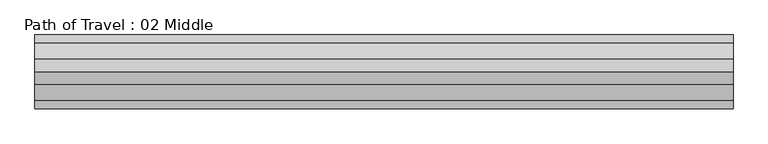
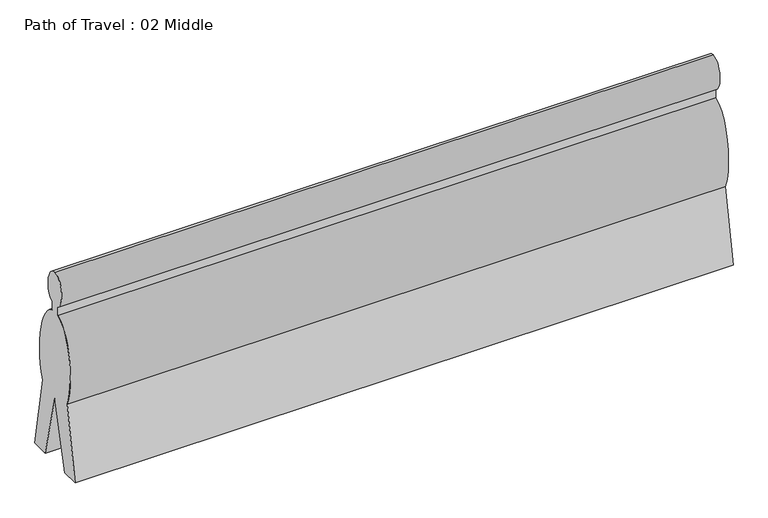
"""IFC4 building model written with IfcOpenShell, lengths in millimetres: proxy geometry, Path of Travel : 02 Middle."""

from ifc_helpers import new_model, si_unit, point, frame, origin, place, context, project, spatial, ellipse_curve, trimmed, source, transform, mapped, element, save
from ifc_brep_helpers import plane_surface, extruded_surface, advanced_brep


def path_of_travel_02_middle_da6d7806(model_context):
    return source(origin(), model_context, "Body", "AdvancedBrep", [
        advanced_brep(
        [(227.5554837, 0.0, 1727.2), (227.5554837, 42.9018657, 1436.6534209), (227.5554837, 42.9018657, 1363.4763406), (227.5554837, 184.1186263, 643.4144547), (227.5554837, 297.5699544, 0.0), (227.5554837, 145.6574193, 0.0), (227.5554837, 0.0, 584.2), (227.5554837, -145.6574193, 0.0), (227.5554837, -297.5699544, 0.0), (227.5554837, -184.1186263, 643.4144547), (227.5554837, -42.9018657, 1363.4763406), (227.5554837, -42.9018657, 1436.6534209), (5866.3554837, 0.0, 1727.2), (5866.3554837, -42.9018657, 1436.6534209), (5866.3554837, -42.9018657, 1363.4763406), (5866.3554837, -184.1186263, 643.4144547), (5866.3554837, -297.5699544, 0.0), (5866.3554837, -145.6574193, 0.0), (5866.3554837, 0.0, 584.2), (5866.3554837, 145.6574193, 0.0), (5866.3554837, 297.5699544, 0.0), (5866.3554837, 184.1186263, 643.4144547), (5866.3554837, 42.9018657, 1363.4763406), (5866.3554837, 42.9018657, 1436.6534209)],
        [
            (0, 1, ellipse_curve(frame((227.5554837, 0.0, 1574.8), z_axis=(-1.0, 0.0, 0.0), x_axis=(0.0, 0.0, 1.0)), 152.4, 101.6)),
            (1, 2),
            (2, 3, ellipse_curve(frame((227.5554837, 0.0, 914.4), z_axis=(-1.0, 0.0, 0.0), x_axis=(0.0, 0.0, -1.0)), 457.2, 228.6)),
            (3, 4),
            (4, 5),
            (5, 6),
            (6, 7),
            (7, 8),
            (8, 9),
            (9, 10, ellipse_curve(frame((227.5554837, 0.0, 914.4), z_axis=(-1.0, 0.0, 0.0), x_axis=(0.0, 0.0, -1.0)), 457.2, 228.6)),
            (10, 11),
            (11, 0, ellipse_curve(frame((227.5554837, 0.0, 1574.8), z_axis=(-1.0, 0.0, 0.0), x_axis=(0.0, 0.0, 1.0)), 152.4, 101.6)),
            (12, 13, ellipse_curve(frame((5866.3554837, 0.0, 1574.8), z_axis=(1.0, 0.0, 0.0), x_axis=(0.0, 0.0, 1.0)), 152.4, 101.6)),
            (13, 14),
            (14, 15, ellipse_curve(frame((5866.3554837, 0.0, 914.4), z_axis=(1.0, 0.0, 0.0), x_axis=(0.0, 0.0, -1.0)), 457.2, 228.6)),
            (15, 16),
            (16, 17),
            (17, 18),
            (18, 19),
            (19, 20),
            (20, 21),
            (21, 22, ellipse_curve(frame((5866.3554837, 0.0, 914.4), z_axis=(1.0, 0.0, 0.0), x_axis=(0.0, 0.0, -1.0)), 457.2, 228.6)),
            (22, 23),
            (23, 12, ellipse_curve(frame((5866.3554837, 0.0, 1574.8), z_axis=(1.0, 0.0, 0.0), x_axis=(0.0, 0.0, 1.0)), 152.4, 101.6)),
            (0, 12),
            (23, 1),
            (22, 2),
            (21, 3),
            (20, 4),
            (19, 5),
            (18, 6),
            (17, 7),
            (16, 8),
            (15, 9),
            (14, 10),
            (13, 11),
        ],
        [
            plane_surface(frame((227.5554837, 0.0, 0.0), z_axis=(-1.0, 0.0, 0.0), x_axis=(0.0, 0.0, 1.0))),
            plane_surface(frame((5866.3554837, 0.0, 0.0), z_axis=(1.0, 0.0, 0.0), x_axis=(0.0, 0.0, 1.0))),
            extruded_surface(trimmed(ellipse_curve(frame((5866.3554837, 0.0, 1574.8), z_axis=(-1.0, 0.0, 0.0), x_axis=(0.0, 0.0, 1.0)), 152.4, 101.6), [point((5866.3554837, 0.0, 1727.2))], [point((5866.3554837, 42.9018657, 1436.6534209))], True, "CARTESIAN"), (-5638.8, 0.0, 0.0), 5638.8),
            plane_surface(frame((227.5554837, 42.9018657, 1436.6534209), z_axis=(0.0, 1.0, 0.0), x_axis=(1.0, 0.0, 0.0))),
            extruded_surface(trimmed(ellipse_curve(frame((5866.3554837, 0.0, 914.4), z_axis=(-1.0, 0.0, 0.0), x_axis=(0.0, 0.0, -1.0)), 457.2, 228.6), [point((5866.3554837, 42.9018657, 1363.4763406))], [point((5866.3554837, 184.1186263, 643.4144547))], True, "CARTESIAN"), (-5638.8, 0.0, 0.0), 5638.8),
            plane_surface(frame((227.5554837, 184.1186263, 643.4144547), z_axis=(0.0, 0.9848077530122078, 0.17364817766693205), x_axis=(1.0, 0.0, 0.0))),
            plane_surface(frame((227.5554837, 297.5699544, 0.0), z_axis=(0.0, 0.0, -1.0), x_axis=(1.0, 0.0, 0.0))),
            plane_surface(frame((227.5554837, 145.6574193, 0.0), z_axis=(0.0, -0.9702957262760199, -0.2419218955995739), x_axis=(1.0, 0.0, 0.0))),
            plane_surface(frame((227.5554837, 0.0, 584.2), z_axis=(0.0, 0.9702957262759961, -0.24192189559966923), x_axis=(1.0, 0.0, 0.0))),
            plane_surface(frame((227.5554837, -145.6574193, 0.0), z_axis=(0.0, 0.0, -1.0), x_axis=(1.0, 0.0, 0.0))),
            plane_surface(frame((227.5554837, -297.5699544, 0.0), z_axis=(0.0, -0.984807753012208, 0.17364817766693066), x_axis=(1.0, 0.0, 0.0))),
            extruded_surface(trimmed(ellipse_curve(frame((5866.3554837, 0.0, 914.4), z_axis=(-1.0, 0.0, 0.0), x_axis=(0.0, 0.0, -1.0)), 457.2, 228.6), [point((5866.3554837, -184.1186263, 643.4144547))], [point((5866.3554837, -42.9018657, 1363.4763406))], True, "CARTESIAN"), (-5638.8, 0.0, 0.0), 5638.8),
            plane_surface(frame((227.5554837, -42.9018657, 1363.4763406), z_axis=(0.0, -1.0, 0.0), x_axis=(1.0, 0.0, 0.0))),
            extruded_surface(trimmed(ellipse_curve(frame((5866.3554837, 0.0, 1574.8), z_axis=(-1.0, 0.0, 0.0), x_axis=(0.0, 0.0, 1.0)), 152.4, 101.6), [point((5866.3554837, -42.9018657, 1436.6534209))], [point((5866.3554837, 0.0, 1727.2))], True, "CARTESIAN"), (-5638.8, 0.0, 0.0), 5638.8),
        ],
        [
            (0, [[1, 2, 3, 4, 5, 6, 7, 8, 9, 10, 11, 12]]),
            (1, [[13, 14, 15, 16, 17, 18, 19, 20, 21, 22, 23, 24]]),
            (2, [[-1, 25, -24, 26]]),
            (3, [[-2, -26, -23, 27]]),
            (4, [[-3, -27, -22, 28]]),
            (5, [[-4, -28, -21, 29]]),
            (6, [[-5, -29, -20, 30]]),
            (7, [[-6, -30, -19, 31]]),
            (8, [[-7, -31, -18, 32]]),
            (9, [[-8, -32, -17, 33]]),
            (10, [[-9, -33, -16, 34]]),
            (11, [[-10, -34, -15, 35]]),
            (12, [[-11, -35, -14, 36]]),
            (13, [[-12, -36, -13, -25]]),
        ],
    ),
    ])


if __name__ == "__main__":
    model = new_model("IFC4")
    model_context = context("Model", 3, world=origin())
    ifc_project = project(units=[si_unit("LENGTHUNIT", "METRE", prefix="MILLI")], contexts=[model_context])
    site = spatial("IfcSite", under=ifc_project)
    building = spatial("IfcBuilding", under=site)
    placement = place(None, origin())
    path_of_travel_02_middle_shape = path_of_travel_02_middle_da6d7806(model_context)
    element("IfcBuildingElementProxy", 1, Name="Path of Travel : 02 Middle", ObjectType="Path of Travel : 02 Middle", at=placement, inside=building, context=model_context, shape_type="MappedRepresentation", body=[
        mapped(path_of_travel_02_middle_shape, transform((0.0, 0.0, 0.0), x_axis=(1.0, 0.0, 0.0), y_axis=(0.0, 1.0, 0.0), z_axis=(0.0, 0.0, 1.0))),
    ])
    save(model, "model.ifc")

# Revit data of these elements
# Type "Path of Travel : 02 Middle"
#   Path of Egress [instance default] = 4' - 0"
#   built-in parameter 1001306 [instance default] = 4 (stored number, unit not read)
#   Dot at Start = no
#   Arrow in Middle = yes
#   Arrow at End = no
#   Egress Path = none
# Element 1 (IfcBuildingElementProxy, "Path of Travel : 02 Middle")
#   Path of Egress = 18' - 6"
#   built-in parameter 1001306 = 18.5 (stored number, unit not read)
#   Materials on its faces: "Egress Path Solid"
# Materials
#   "Egress Path Solid": class "Unassigned", colour RGB 255 128 64, transparency 0.75, Comments = "Rendering appearance not upgraded "
